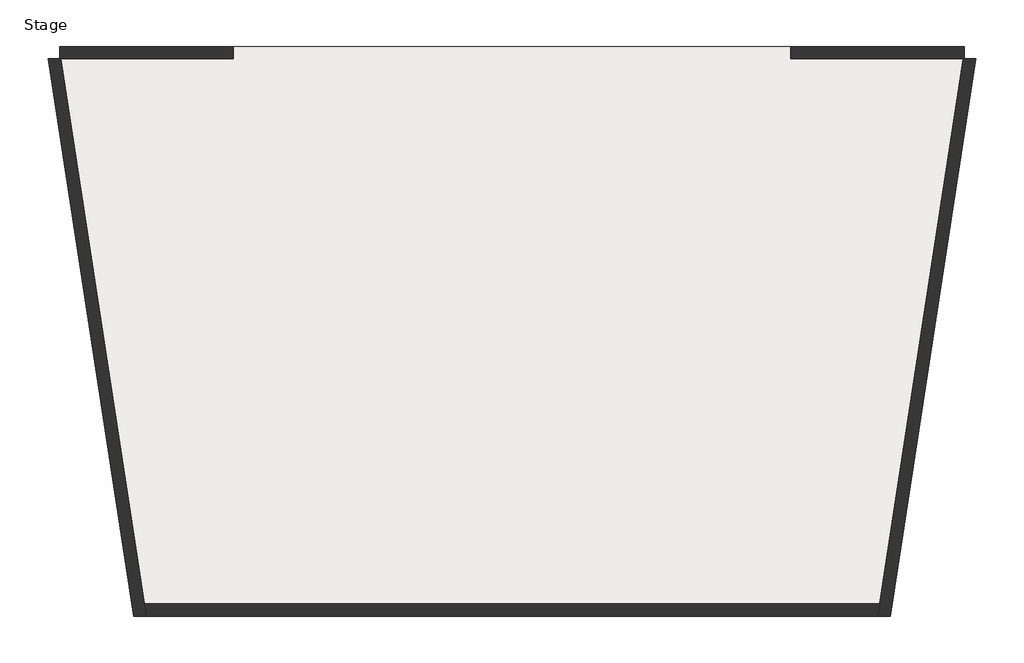
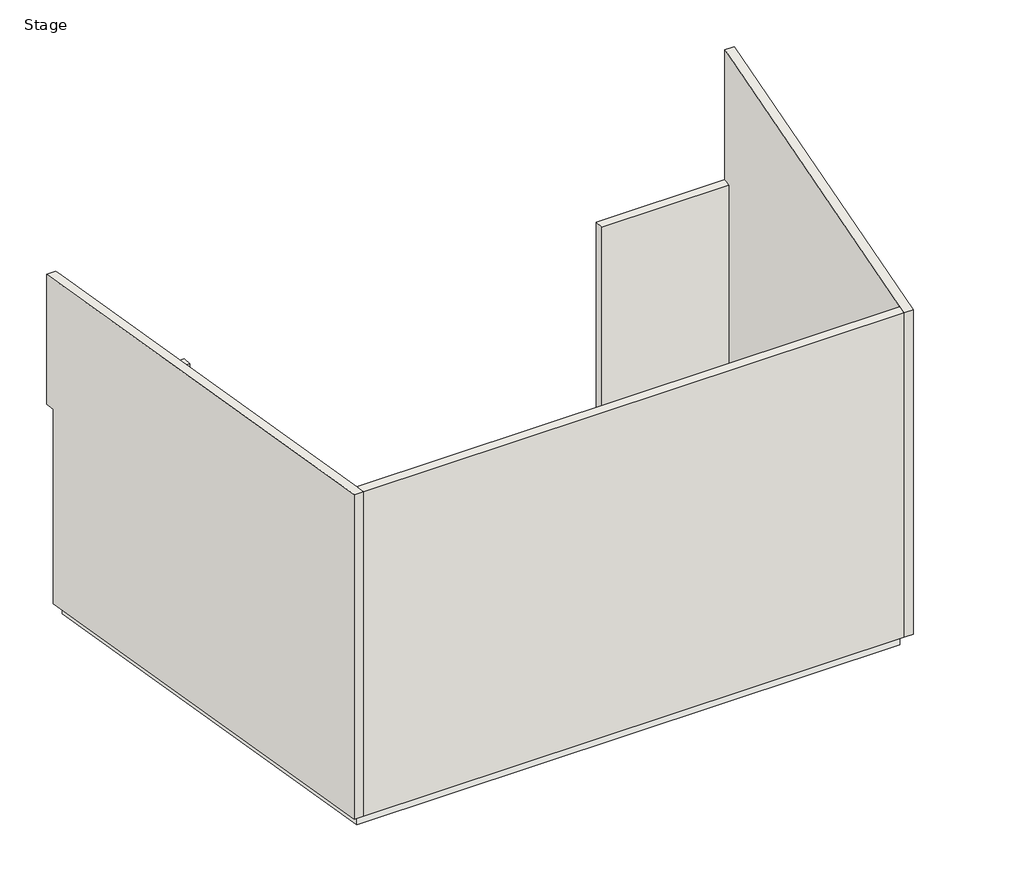
# One storey: 5 walls, 1 slab.
"""IFC4 building model written with IfcOpenShell, lengths in millimetres."""

from ifc_helpers import new_model, si_unit, frame, origin, place, context, project, spatial, polyline, outline, extrude, faceted_brep, element, save

model = new_model("IFC4")

# Units and contexts
model_context = context("Model", 3, world=origin())
ifc_project = project(units=[si_unit("LENGTHUNIT", "METRE", prefix="MILLI")], contexts=[model_context])

# Site, building, storey
site = spatial("IfcSite", under=ifc_project)
building = spatial("IfcBuilding", under=site)
storey = spatial("IfcBuildingStorey", under=building, Name="Stage", Elevation=1524.0)

# Slab
placement = place(None, origin())
element("IfcSlab", 1, ObjectType="Generic - 12\"", at=placement, inside=storey, context=model_context, shape_type="SweptSolid", body=[
    extrude(outline(polyline([(36633.2673832, -6049.3470145), (36633.2673832, -5846.1470145), (45777.2673832, -5846.1470145), (45777.2673832, -6049.3470145), (48596.9349665, -6049.3470145), (47230.4174982, -14990.1470145), (35180.1266506, -14990.1470145), (33813.5999211, -6049.3470145), (36633.2673832, -6049.3470145)])), frame((0.0, 0.0, 1219.2), z_axis=(0.0, 0.0, 1.0), x_axis=(1.0, 0.0, 0.0)), (0.0, 0.0, 1.0), 304.8),
])

# Walls
element("IfcWall", 2, ObjectType="Generic - 8\"", at=placement, inside=storey, context=model_context, shape_type="Brep", body=[
    faceted_brep([(48613.6434245, -5846.1470145, 1524.0), (45777.2673832, -5846.1470145, 1524.0), (45777.2673832, -5846.1470145, 6096.0), (48613.6434245, -5846.1470145, 6096.0), (48613.6434245, -6049.3470145, 1524.0), (48613.6434245, -6049.3470145, 6096.0), (48596.9349665, -6049.3470145, 6096.0), (45777.2673832, -6049.3470145, 6096.0), (45777.2673832, -6049.3470145, 1524.0), (48596.9349665, -6049.3470145, 1524.0)], [[[0, 1, 2, 3]], [[4, 5, 6, 7, 8, 9]], [[1, 0, 4, 9, 8]], [[2, 1, 8, 7]], [[3, 2, 7, 6, 5]], [[0, 3, 5, 4]]]),
])
element("IfcWall", 3, ObjectType="Generic - 8\"", at=placement, inside=storey, context=model_context, shape_type="Brep", body=[
    faceted_brep([(48596.9349665, -6049.3470145, 1524.0), (47230.4174982, -14990.1470145, 1524.0), (47199.360283, -15193.3470145, 1524.0), (47199.360283, -15193.3470145, 9144.0), (47230.4174982, -14990.1470145, 9144.0), (48596.9349665, -6049.3470145, 9144.0), (48627.9921817, -5846.1470145, 9144.0), (48627.9921817, -5846.1470145, 6096.0), (48596.9349665, -6049.3470145, 6096.0), (48802.4946674, -6049.3470145, 1524.0), (48802.4946674, -6049.3470145, 6096.0), (48833.5518826, -5846.1470145, 6096.0), (48833.5518826, -5846.1470145, 9144.0), (47404.9199839, -15193.3470145, 9144.0), (47404.9199839, -15193.3470145, 1524.0), (48613.6434245, -6049.3470145, 1524.0), (48613.6434245, -6049.3470145, 6096.0)], [[[0, 1, 2, 3, 4, 5, 6, 7, 8]], [[9, 10, 11, 12, 13, 14]], [[2, 1, 0, 15, 9, 14]], [[6, 5, 4, 3, 13, 12]], [[3, 2, 14, 13]], [[7, 11, 10, 16, 8]], [[0, 8, 16, 10, 9, 15]], [[7, 6, 12, 11]]]),
])
element("IfcWall", 4, ObjectType="Generic - 8\"", at=placement, inside=storey, context=model_context, shape_type="SweptSolid", body=[
    extrude(outline(polyline([(35180.1266506, -14990.1470145), (47230.4174982, -14990.1470145), (47199.360283, -15193.3470145), (35211.1840762, -15193.3470145), (35180.1266506, -14990.1470145)])), frame((0.0, 0.0, 1524.0), z_axis=(0.0, 0.0, 1.0), x_axis=(1.0, 0.0, 0.0)), (0.0, 0.0, 1.0), 7620.0),
])
element("IfcWall", 5, ObjectType="Generic - 8\"", at=placement, inside=storey, context=model_context, shape_type="Brep", body=[
    faceted_brep([(33796.891342, -6049.3470145, 1524.0), (33813.5999211, -6049.3470145, 1524.0), (36633.2673832, -6049.3470145, 1524.0), (36633.2673832, -6049.3470145, 6096.0), (33813.5999211, -6049.3470145, 6096.0), (33796.891342, -6049.3470145, 6096.0), (33796.891342, -5846.1470145, 1524.0), (33796.891342, -5846.1470145, 6096.0), (36633.2673832, -5846.1470145, 6096.0), (36633.2673832, -5846.1470145, 1524.0)], [[[0, 1, 2, 3, 4, 5]], [[6, 7, 8, 9]], [[2, 1, 0, 6, 9]], [[3, 2, 9, 8]], [[5, 4, 3, 8, 7]], [[0, 5, 7, 6]]]),
])
element("IfcWall", 6, ObjectType="Generic - 8\"", at=placement, inside=storey, context=model_context, shape_type="Brep", body=[
    faceted_brep([(33608.0401885, -6049.3470145, 1524.0), (35005.6243436, -15193.3470145, 1524.0), (35005.6243436, -15193.3470145, 9144.0), (33576.9827628, -5846.1470145, 9144.0), (33576.9827628, -5846.1470145, 6096.0), (33608.0401885, -6049.3470145, 6096.0), (33813.5999211, -6049.3470145, 1524.0), (33813.5999211, -6049.3470145, 6096.0), (33782.5424954, -5846.1470145, 6096.0), (33782.5424954, -5846.1470145, 9144.0), (33813.5999211, -6049.3470145, 9144.0), (35180.1266506, -14990.1470145, 9144.0), (35211.1840762, -15193.3470145, 9144.0), (35211.1840762, -15193.3470145, 1524.0), (35180.1266506, -14990.1470145, 1524.0), (33796.891342, -6049.3470145, 1524.0), (33796.891342, -6049.3470145, 6096.0)], [[[0, 1, 2, 3, 4, 5]], [[6, 7, 8, 9, 10, 11, 12, 13, 14]], [[1, 0, 15, 6, 14, 13]], [[3, 2, 12, 11, 10, 9]], [[2, 1, 13, 12]], [[4, 8, 7, 16, 5]], [[0, 5, 16, 7, 6, 15]], [[4, 3, 9, 8]]]),
])

save(model, "model.ifc")

# Revit data of these elements
# Type "Generic - 12\""
#   Assembly Code = "B1010"
#   Function = 0
#   Layers, outside or top first: 1' - 0" no material (function 1)
# Type "Generic - 8\""
#   Assembly Code = "B2010"
#   Layers, outside or top first: 0' - 8" no material (function 1)
# Element 1 (IfcSlab, "Generic - 12\"")
#   Height Offset From Level = 0' - 0"
#   Phase Created = New Construction
#   Materials on its faces: "Default Floor"
# Elements 2, 5 (IfcWall, "Generic - 8\"")
#   Top Offset = 0' - 0"
#   Base Offset = 0' - 0"
#   wall height = 15' - 0"
#   Phase Created = New Construction
#   Base Constraint = Stage
#   Top Constraint = Level 3
#   Materials on its faces: "Default Wall"
# Elements 3, 4, 6 (IfcWall, "Generic - 8\"")
#   Top Offset = 0' - 0"
#   Base Offset = 0' - 0"
#   wall height = 25' - 0"
#   Phase Created = New Construction
#   Base Constraint = Stage
#   Top Constraint = Level 4
#   Materials on its faces: "Default Wall"
# Materials
#   "Default Floor": class "Miscellaneous", colour RGB 128 128 128, transparency 0, Cost = 0
#   "Default Wall": class "Miscellaneous", colour RGB 128 128 128, transparency 0, Cost = 0
# Room at (41042.888, -9537.834) mm, phase "New Construction", upper level "Level 4", upper offset 10' - 0", lower offset 0' - 0"
#   Number = "10018"
#   Name = "Stage"
